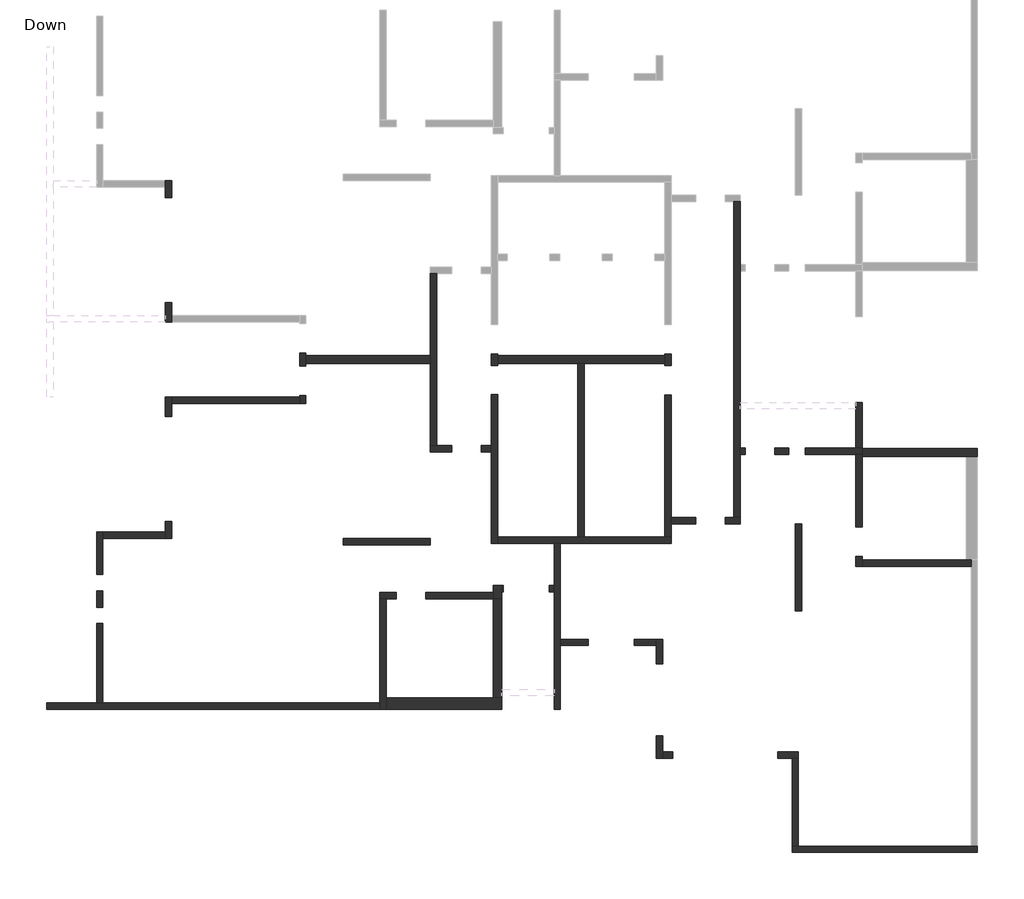
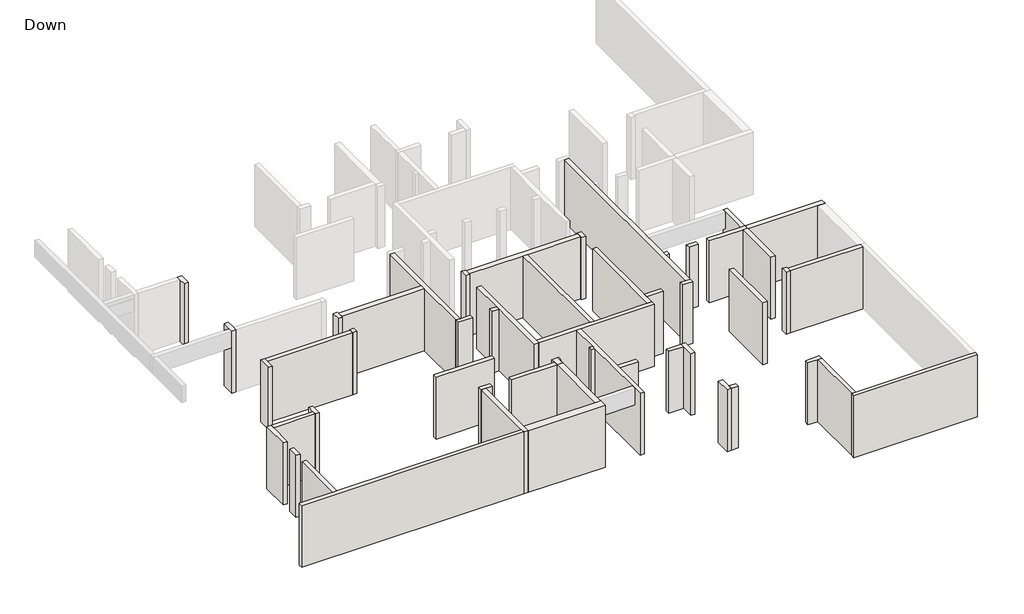
# One storey, part 1 of 2: 53 walls.
"""IFC4 building model written with IfcOpenShell, lengths in millimetres."""

from ifc_helpers import new_model, si_unit, origin, place, context, project, spatial, faceted_brep, element, save

model = new_model("IFC4")

# Units and contexts
model_context = context("Model", 3, world=origin())
ifc_project = project(units=[si_unit("LENGTHUNIT", "METRE", prefix="MILLI")], contexts=[model_context])

# Site, building, storey
site = spatial("IfcSite", under=ifc_project)
building = spatial("IfcBuilding", under=site)
storey = spatial("IfcBuildingStorey", under=building, Name="Down", Elevation=0.0)

# Walls
placement = place(None, origin())
element("IfcWall", 1, ObjectType="19", at=placement, inside=storey, context=model_context, shape_type="Brep", body=[
    faceted_brep([(7776.7577342, 20248.0459905, 0.0), (7776.7577342, 20058.0459905, 0.0), (7776.7577342, 19727.6893828, 0.0), (7776.7577342, 19727.6893828, 2810.0), (7776.7577342, 19727.6893828, 3000.0), (7776.7577342, 20058.0459905, 3000.0), (7776.7577342, 20248.0459905, 3000.0), (7966.7577342, 20248.0459905, 0.0), (7966.7577342, 20248.0459905, 2810.0), (7966.7577342, 20248.0459905, 3000.0), (7966.7577342, 19727.6893828, 3000.0), (7966.7577342, 19727.6893828, 2810.0), (7966.7577342, 19727.6893828, 0.0)], [[[0, 1, 2, 3, 4, 5, 6]], [[7, 8, 9, 10, 11, 12]], [[2, 1, 0, 7, 12]], [[4, 3, 2, 12, 11, 10]], [[6, 5, 4, 10, 9]], [[0, 6, 9, 8, 7]]]),
])
element("IfcWall", 2, ObjectType="19", at=placement, inside=storey, context=model_context, shape_type="Brep", body=[
    faceted_brep([(7776.7577342, 16527.889163, 0.0), (7776.7577342, 15926.4707233, 0.0), (7776.7577342, 15926.4707233, 3000.0), (7776.7577342, 16126.4707233, 3000.0), (7776.7577342, 16527.889163, 3000.0), (7776.7577342, 16527.889163, 2810.0), (7966.7577342, 16527.889163, 0.0), (7966.7577342, 16527.889163, 2810.0), (7966.7577342, 16527.889163, 3000.0), (7966.7577342, 16126.4707233, 3000.0), (7966.7577342, 15926.4707233, 3000.0), (7966.7577342, 15926.4707233, 0.0), (7966.7577342, 16126.4707233, 0.0)], [[[0, 1, 2, 3, 4, 5]], [[6, 7, 8, 9, 10, 11, 12]], [[1, 0, 6, 12, 11]], [[4, 3, 2, 10, 9, 8]], [[0, 5, 4, 8, 7, 6]], [[2, 1, 11, 10]]]),
])
element("IfcWall", 3, ObjectType="19", at=placement, inside=storey, context=model_context, shape_type="Brep", body=[
    faceted_brep([(11878.6856136, 14975.6366408, 0.0), (11878.6856136, 14585.9852573, 0.0), (11878.6856136, 14585.9852573, 2810.0), (11878.6856136, 14585.9852573, 3000.0), (11878.6856136, 14975.6366408, 3000.0), (11878.6856136, 14975.6366408, 2810.0), (12068.6856136, 14975.6366408, 0.0), (12068.6856136, 14975.6366408, 2810.0), (12068.6856136, 14975.6366408, 3000.0), (12068.6856136, 14905.7535122, 3000.0), (12068.6856136, 14655.7535122, 3000.0), (12068.6856136, 14585.9852573, 3000.0), (12068.6856136, 14585.9852573, 2810.0), (12068.6856136, 14585.9852573, 0.0), (12068.6856136, 14655.7535122, 0.0), (12068.6856136, 14905.7535122, 0.0)], [[[0, 1, 2, 3, 4, 5]], [[6, 7, 8, 9, 10, 11, 12, 13, 14, 15]], [[1, 0, 6, 15, 14, 13]], [[3, 2, 1, 13, 12, 11]], [[4, 3, 11, 10, 9, 8]], [[0, 5, 4, 8, 7, 6]]]),
])
element("IfcWall", 4, ObjectType="19", at=placement, inside=storey, context=model_context, shape_type="Brep", body=[
    faceted_brep([(32597.3840453, -100.765317, 0.0), (32407.3840453, -100.765317, 0.0), (27124.7329615, -100.765317, 0.0), (26934.7329615, -100.765317, 0.0), (26934.7329615, -100.765317, 3000.0), (27124.7329615, -100.765317, 3000.0), (32407.3840453, -100.765317, 3000.0), (32597.3840453, -100.765317, 3000.0), (32597.3840453, -290.765317, 0.0), (32597.3840453, -290.765317, 3000.0), (26934.7329615, -290.765317, 3000.0), (26934.7329615, -290.765317, 2810.0), (26934.7329615, -290.765317, 0.0)], [[[0, 1, 2, 3, 4, 5, 6, 7]], [[8, 9, 10, 11, 12]], [[3, 2, 1, 0, 8, 12]], [[7, 6, 5, 4, 10, 9]], [[4, 3, 12, 11, 10]], [[0, 7, 9, 8]]]),
])
element("IfcWall", 5, ObjectType="19", at=placement, inside=storey, context=model_context, shape_type="Brep", body=[
    faceted_brep([(14329.4188071, 4280.8870961, 0.0), (5866.0285364, 4280.8870961, 0.0), (5676.0285364, 4280.8870961, 0.0), (4143.9417549, 4280.8870961, 0.0), (4143.9417549, 4280.8870961, 3000.0), (4344.3623691, 4280.8870961, 3000.0), (5676.0285364, 4280.8870961, 3000.0), (5866.0285364, 4280.8870961, 3000.0), (14329.4188071, 4280.8870961, 3000.0), (14329.4188071, 4280.8870961, 2810.0), (14329.4188071, 4090.8870961, 0.0), (14329.4188071, 4090.8870961, 3000.0), (4143.9417549, 4090.8870961, 3000.0), (4143.9417549, 4090.8870961, 0.0)], [[[0, 1, 2, 3, 4, 5, 6, 7, 8, 9]], [[10, 11, 12, 13]], [[3, 2, 1, 0, 10, 13]], [[4, 3, 13, 12]], [[8, 7, 6, 5, 4, 12, 11]], [[0, 9, 8, 11, 10]]]),
])
element("IfcWall", 6, ObjectType="19", at=placement, inside=storey, context=model_context, shape_type="Brep", body=[
    faceted_brep([(5866.0285364, 4280.8870961, 0.0), (5866.0285364, 6709.6372401, 0.0), (5866.0285364, 6709.6372401, 2810.0), (5866.0285364, 6709.6372401, 3000.0), (5866.0285364, 4280.8870961, 3000.0), (5866.0285364, 4280.8870961, 2810.0), (5676.0285364, 4280.8870961, 0.0), (5676.0285364, 4280.8870961, 2810.0), (5676.0285364, 4280.8870961, 3000.0), (5676.0285364, 6709.6372401, 3000.0), (5676.0285364, 6709.6372401, 2810.0), (5676.0285364, 6709.6372401, 0.0)], [[[0, 1, 2, 3, 4, 5]], [[6, 7, 8, 9, 10, 11]], [[1, 0, 6, 11]], [[3, 2, 1, 11, 10, 9]], [[4, 3, 9, 8]], [[0, 5, 4, 8, 7, 6]]]),
])
element("IfcWall", 7, ObjectType="19", at=placement, inside=storey, context=model_context, shape_type="Brep", body=[
    faceted_brep([(5866.0285364, 7208.8680094, 0.0), (5866.0285364, 7708.0987786, 0.0), (5866.0285364, 7708.0987786, 2810.0), (5866.0285364, 7708.0987786, 3000.0), (5866.0285364, 7208.8680094, 3000.0), (5866.0285364, 7208.8680094, 2810.0), (5676.0285364, 7208.8680094, 0.0), (5676.0285364, 7208.8680094, 2810.0), (5676.0285364, 7208.8680094, 3000.0), (5676.0285364, 7708.0987786, 3000.0), (5676.0285364, 7708.0987786, 2810.0), (5676.0285364, 7708.0987786, 0.0)], [[[0, 1, 2, 3, 4, 5]], [[6, 7, 8, 9, 10, 11]], [[1, 0, 6, 11]], [[3, 2, 1, 11, 10, 9]], [[4, 3, 9, 8]], [[0, 5, 4, 8, 7, 6]]]),
])
element("IfcWall", 8, ObjectType="19", at=placement, inside=storey, context=model_context, shape_type="Brep", body=[
    faceted_brep([(5866.0285364, 8207.3295478, 0.0), (5866.0285364, 9313.461034, 0.0), (5866.0285364, 9503.461034, 0.0), (5866.0285364, 9503.461034, 3000.0), (5866.0285364, 9313.461034, 3000.0), (5866.0285364, 8207.3295478, 3000.0), (5866.0285364, 8207.3295478, 2810.0), (5676.0285364, 8207.3295478, 0.0), (5676.0285364, 8207.3295478, 2810.0), (5676.0285364, 8207.3295478, 3000.0), (5676.0285364, 9308.461034, 3000.0), (5676.0285364, 9503.461034, 3000.0), (5676.0285364, 9503.461034, 0.0)], [[[0, 1, 2, 3, 4, 5, 6]], [[7, 8, 9, 10, 11, 12]], [[2, 1, 0, 7, 12]], [[5, 4, 3, 11, 10, 9]], [[0, 6, 5, 9, 8, 7]], [[3, 2, 12, 11]]]),
])
element("IfcWall", 9, ObjectType="19", at=placement, inside=storey, context=model_context, shape_type="Brep", body=[
    faceted_brep([(27124.7329615, -100.765317, 0.0), (27124.7329615, 2589.8569984, 0.0), (27124.7329615, 2589.8569984, 3000.0), (27124.7329615, -100.765317, 3000.0), (27124.7329615, -100.765317, 2810.0), (26934.7329615, -100.765317, 0.0), (26934.7329615, -100.765317, 3000.0), (26934.7329615, 2589.8569984, 3000.0), (26934.7329615, 2589.8569984, 2810.0), (26934.7329615, 2589.8569984, 0.0)], [[[0, 1, 2, 3, 4]], [[5, 6, 7, 8, 9]], [[1, 0, 5, 9]], [[3, 2, 7, 6]], [[0, 4, 3, 6, 5]], [[2, 1, 9, 8, 7]]]),
])
element("IfcWall", 10, ObjectType="19", at=placement, inside=storey, context=model_context, shape_type="Brep", body=[
    faceted_brep([(27124.7329615, 2779.8569984, 0.0), (26490.0221434, 2779.8569984, 0.0), (26490.0221434, 2779.8569984, 2810.0), (26490.0221434, 2779.8569984, 3000.0), (27124.7329615, 2779.8569984, 3000.0), (27124.7329615, 2779.8569984, 2810.0), (27124.7329615, 2589.8569984, 0.0), (27124.7329615, 2589.8569984, 3000.0), (26934.7329615, 2589.8569984, 3000.0), (26490.0221434, 2589.8569984, 3000.0), (26490.0221434, 2589.8569984, 2810.0), (26490.0221434, 2589.8569984, 0.0), (26934.7329615, 2589.8569984, 0.0)], [[[0, 1, 2, 3, 4, 5]], [[6, 7, 8, 9, 10, 11, 12]], [[1, 0, 6, 12, 11]], [[3, 2, 1, 11, 10, 9]], [[4, 3, 9, 8, 7]], [[0, 5, 4, 7, 6]]]),
])
element("IfcWall", 11, ObjectType="19", at=placement, inside=storey, context=model_context, shape_type="Brep", body=[
    faceted_brep([(23288.1042531, 2779.8569984, 0.0), (22974.0986592, 2779.8569984, 0.0), (22974.0986592, 2779.8569984, 2810.0), (22974.0986592, 2779.8569984, 3000.0), (23288.1042531, 2779.8569984, 3000.0), (23288.1042531, 2779.8569984, 2810.0), (23288.1042531, 2589.8569984, 0.0), (23288.1042531, 2589.8569984, 2810.0), (23288.1042531, 2589.8569984, 3000.0), (22974.0986592, 2589.8569984, 3000.0), (22974.0986592, 2589.8569984, 0.0)], [[[0, 1, 2, 3, 4, 5]], [[6, 7, 8, 9, 10]], [[1, 0, 6, 10]], [[4, 3, 9, 8]], [[0, 5, 4, 8, 7, 6]], [[3, 2, 1, 10, 9]]]),
])
element("IfcWall", 12, ObjectType="19", at=placement, inside=storey, context=model_context, shape_type="Brep", body=[
    faceted_brep([(22974.0986592, 2589.8569984, 0.0), (22974.0986592, 2779.8569984, 0.0), (22974.0986592, 3279.6272511, 0.0), (22974.0986592, 3279.6272511, 2810.0), (22974.0986592, 3279.6272511, 3000.0), (22974.0986592, 2779.8569984, 3000.0), (22974.0986592, 2589.8569984, 3000.0), (22784.0986592, 2589.8569984, 0.0), (22784.0986592, 2589.8569984, 2810.0), (22784.0986592, 2589.8569984, 3000.0), (22784.0986592, 3279.6272511, 3000.0), (22784.0986592, 3279.6272511, 2810.0), (22784.0986592, 3279.6272511, 0.0)], [[[0, 1, 2, 3, 4, 5, 6]], [[7, 8, 9, 10, 11, 12]], [[2, 1, 0, 7, 12]], [[4, 3, 2, 12, 11, 10]], [[6, 5, 4, 10, 9]], [[0, 6, 9, 8, 7]]]),
])
element("IfcWall", 13, ObjectType="19", at=placement, inside=storey, context=model_context, shape_type="Brep", body=[
    faceted_brep([(22974.6890098, 5479.8869654, 0.0), (22974.6890098, 6231.6600151, 0.0), (22974.6890098, 6231.6600151, 2810.0), (22974.6890098, 6231.6600151, 3000.0), (22974.6890098, 5479.8869654, 3000.0), (22974.6890098, 5479.8869654, 2810.0), (22784.6890098, 5479.8869654, 0.0), (22784.6890098, 5479.8869654, 2810.0), (22784.6890098, 5479.8869654, 3000.0), (22784.6890098, 6041.6600151, 3000.0), (22784.6890098, 6231.6600151, 3000.0), (22784.6890098, 6231.6600151, 0.0), (22784.6890098, 6041.6600151, 0.0)], [[[0, 1, 2, 3, 4, 5]], [[6, 7, 8, 9, 10, 11, 12]], [[1, 0, 6, 12, 11]], [[4, 3, 10, 9, 8]], [[0, 5, 4, 8, 7, 6]], [[3, 2, 1, 11, 10]]]),
])
element("IfcWall", 14, ObjectType="19", at=placement, inside=storey, context=model_context, shape_type="Brep", body=[
    faceted_brep([(22784.6890098, 6231.6600151, 0.0), (22104.3264087, 6231.6600151, 0.0), (22104.3264087, 6231.6600151, 2810.0), (22104.3264087, 6231.6600151, 3000.0), (22784.6890098, 6231.6600151, 3000.0), (22784.6890098, 6041.6600151, 0.0), (22784.6890098, 6041.6600151, 2810.0), (22784.6890098, 6041.6600151, 3000.0), (22104.3264087, 6041.6600151, 3000.0), (22104.3264087, 6041.6600151, 2810.0), (22104.3264087, 6041.6600151, 0.0)], [[[0, 1, 2, 3, 4]], [[5, 6, 7, 8, 9, 10]], [[1, 0, 5, 10]], [[3, 2, 1, 10, 9, 8]], [[4, 3, 8, 7]], [[0, 4, 7, 6, 5]]]),
])
element("IfcWall", 15, ObjectType="19", at=placement, inside=storey, context=model_context, shape_type="Brep", body=[
    faceted_brep([(20702.4284964, 6231.6600151, 0.0), (19852.6522503, 6231.6600151, 0.0), (19852.6522503, 6231.6600151, 2810.0), (19852.6522503, 6231.6600151, 3000.0), (20702.4284964, 6231.6600151, 3000.0), (20702.4284964, 6231.6600151, 2810.0), (20702.4284964, 6041.6600151, 0.0), (20702.4284964, 6041.6600151, 2810.0), (20702.4284964, 6041.6600151, 3000.0), (19852.6522503, 6041.6600151, 3000.0), (19852.6522503, 6041.6600151, 2810.0), (19852.6522503, 6041.6600151, 0.0)], [[[0, 1, 2, 3, 4, 5]], [[6, 7, 8, 9, 10, 11]], [[1, 0, 6, 11]], [[4, 3, 9, 8]], [[0, 5, 4, 8, 7, 6]], [[3, 2, 1, 11, 10, 9]]]),
])
element("IfcWall", 16, ObjectType="19", at=placement, inside=storey, context=model_context, shape_type="Brep", body=[
    faceted_brep([(19662.6522503, 9151.9277206, 0.0), (19662.6522503, 7872.8547009, 0.0), (19662.6522503, 7682.8547009, 0.0), (19662.6522503, 4090.6950765, 0.0), (19662.6522503, 4090.6950765, 2810.0), (19662.6522503, 4090.6950765, 3000.0), (19662.6522503, 4692.2283899, 3000.0), (19662.6522503, 7682.8547009, 3000.0), (19662.6522503, 7872.8547009, 3000.0), (19662.6522503, 9151.9277206, 3000.0), (19662.6522503, 9151.9277206, 2810.0), (19852.6522503, 9151.9277206, 0.0), (19852.6522503, 9151.9277206, 2810.0), (19852.6522503, 9151.9277206, 3000.0), (19852.6522503, 6231.6600151, 3000.0), (19852.6522503, 6041.6600151, 3000.0), (19852.6522503, 4090.6950765, 3000.0), (19852.6522503, 4090.6950765, 2810.0), (19852.6522503, 4090.6950765, 0.0), (19852.6522503, 6041.6600151, 0.0), (19852.6522503, 6231.6600151, 0.0)], [[[0, 1, 2, 3, 4, 5, 6, 7, 8, 9, 10]], [[11, 12, 13, 14, 15, 16, 17, 18, 19, 20]], [[3, 2, 1, 0, 11, 20, 19, 18]], [[5, 4, 3, 18, 17, 16]], [[9, 8, 7, 6, 5, 16, 15, 14, 13]], [[0, 10, 9, 13, 12, 11]]]),
])
element("IfcWall", 17, ObjectType="19", at=placement, inside=storey, context=model_context, shape_type="Brep", body=[
    faceted_brep([(5866.0285364, 9313.461034, 0.0), (7776.7577342, 9313.461034, 0.0), (7776.7577342, 9313.461034, 3000.0), (5866.0285364, 9313.461034, 3000.0), (5866.0285364, 9313.461034, 2810.0), (5866.0285364, 9503.461034, 0.0), (5866.0285364, 9503.461034, 3000.0), (7776.7577342, 9503.461034, 3000.0), (7776.7577342, 9503.461034, 2810.0), (7776.7577342, 9503.461034, 0.0)], [[[0, 1, 2, 3, 4]], [[5, 6, 7, 8, 9]], [[1, 0, 5, 9]], [[3, 2, 7, 6]], [[0, 4, 3, 6, 5]], [[2, 1, 9, 8, 7]]]),
])
element("IfcWall", 18, ObjectType="19", at=placement, inside=storey, context=model_context, shape_type="Brep", body=[
    faceted_brep([(7966.7577342, 9313.461034, 0.0), (7966.7577342, 9833.8176417, 0.0), (7966.7577342, 9833.8176417, 2810.0), (7966.7577342, 9833.8176417, 3000.0), (7966.7577342, 9313.461034, 3000.0), (7966.7577342, 9313.461034, 2810.0), (7776.7577342, 9313.461034, 0.0), (7776.7577342, 9313.461034, 3000.0), (7776.7577342, 9503.461034, 3000.0), (7776.7577342, 9833.8176417, 3000.0), (7776.7577342, 9833.8176417, 2810.0), (7776.7577342, 9833.8176417, 0.0), (7776.7577342, 9503.461034, 0.0)], [[[0, 1, 2, 3, 4, 5]], [[6, 7, 8, 9, 10, 11, 12]], [[1, 0, 6, 12, 11]], [[3, 2, 1, 11, 10, 9]], [[4, 3, 9, 8, 7]], [[0, 5, 4, 7, 6]]]),
])
element("IfcWall", 19, ObjectType="19", at=placement, inside=storey, context=model_context, shape_type="Brep", body=[
    faceted_brep([(7966.7577342, 13033.6178615, 0.0), (7966.7577342, 13435.0363012, 0.0), (7966.7577342, 13635.0363012, 0.0), (7966.7577342, 13635.0363012, 3000.0), (7966.7577342, 13435.0363012, 3000.0), (7966.7577342, 13033.6178615, 3000.0), (7966.7577342, 13033.6178615, 2810.0), (7776.7577342, 13033.6178615, 0.0), (7776.7577342, 13033.6178615, 2810.0), (7776.7577342, 13033.6178615, 3000.0), (7776.7577342, 13435.0363012, 3000.0), (7776.7577342, 13635.0363012, 3000.0), (7776.7577342, 13635.0363012, 0.0)], [[[0, 1, 2, 3, 4, 5, 6]], [[7, 8, 9, 10, 11, 12]], [[2, 1, 0, 7, 12]], [[5, 4, 3, 11, 10, 9]], [[0, 6, 5, 9, 8, 7]], [[3, 2, 12, 11]]]),
])
element("IfcWall", 20, ObjectType="19", at=placement, inside=storey, context=model_context, shape_type="Brep", body=[
    faceted_brep([(12068.6856136, 13435.0363012, 0.0), (12068.6856136, 13683.7427241, 0.0), (12068.6856136, 13683.7427241, 2810.0), (12068.6856136, 13683.7427241, 3000.0), (12068.6856136, 13435.0363012, 3000.0), (12068.6856136, 13435.0363012, 2810.0), (11878.6856136, 13435.0363012, 0.0), (11878.6856136, 13435.0363012, 3000.0), (11878.6856136, 13635.0363012, 3000.0), (11878.6856136, 13683.7427241, 3000.0), (11878.6856136, 13683.7427241, 2810.0), (11878.6856136, 13683.7427241, 0.0), (11878.6856136, 13635.0363012, 0.0)], [[[0, 1, 2, 3, 4, 5]], [[6, 7, 8, 9, 10, 11, 12]], [[1, 0, 6, 12, 11]], [[3, 2, 1, 11, 10, 9]], [[4, 3, 9, 8, 7]], [[0, 5, 4, 7, 6]]]),
])
element("IfcWall", 21, ObjectType="19", at=placement, inside=storey, context=model_context, shape_type="Brep", body=[
    faceted_brep([(18051.1049523, 7682.8547009, 0.0), (18101.9290458, 7682.8547009, 0.0), (18101.9290458, 7682.8547009, 2810.0), (18101.9290458, 7682.8547009, 3000.0), (18051.1049523, 7682.8547009, 3000.0), (18051.1049523, 7682.8547009, 2810.0), (18051.1049523, 7872.8547009, 0.0), (18051.1049523, 7872.8547009, 3000.0), (18101.9290458, 7872.8547009, 3000.0), (18101.9290458, 7872.8547009, 2810.0), (18101.9290458, 7872.8547009, 0.0)], [[[0, 1, 2, 3, 4, 5]], [[6, 7, 8, 9, 10]], [[1, 0, 6, 10]], [[3, 2, 1, 10, 9, 8]], [[4, 3, 8, 7]], [[0, 5, 4, 7, 6]]]),
])
element("IfcWall", 22, ObjectType="19", at=placement, inside=storey, context=model_context, shape_type="Brep", body=[
    faceted_brep([(19501.7092875, 7682.8547009, 0.0), (19662.6522503, 7682.8547009, 0.0), (19662.6522503, 7682.8547009, 2810.0), (19662.6522503, 7682.8547009, 3000.0), (19501.7092875, 7682.8547009, 3000.0), (19501.7092875, 7682.8547009, 2810.0), (19501.7092875, 7872.8547009, 0.0), (19501.7092875, 7872.8547009, 2810.0), (19501.7092875, 7872.8547009, 3000.0), (19662.6522503, 7872.8547009, 3000.0), (19662.6522503, 7872.8547009, 2810.0), (19662.6522503, 7872.8547009, 0.0)], [[[0, 1, 2, 3, 4, 5]], [[6, 7, 8, 9, 10, 11]], [[1, 0, 6, 11]], [[4, 3, 9, 8]], [[0, 5, 4, 8, 7, 6]], [[3, 2, 1, 11, 10, 9]]]),
])
element("IfcWall", 23, ObjectType="20", at=placement, inside=storey, context=model_context, shape_type="Brep", body=[
    faceted_brep([(23033.0448184, 14956.5776057, 0.0), (23033.0448184, 14905.8683859, 0.0), (23033.0448184, 14655.8683859, 0.0), (23033.0448184, 14596.5776057, 0.0), (23033.0448184, 14596.5776057, 2810.0), (23033.0448184, 14596.5776057, 3000.0), (23033.0448184, 14655.8683859, 3000.0), (23033.0448184, 14905.8683859, 3000.0), (23033.0448184, 14956.5776057, 3000.0), (23033.0448184, 14956.5776057, 2810.0), (23233.0448184, 14956.5776057, 0.0), (23233.0448184, 14956.5776057, 2810.0), (23233.0448184, 14956.5776057, 3000.0), (23233.0448184, 14596.5776057, 3000.0), (23233.0448184, 14596.5776057, 2810.0), (23233.0448184, 14596.5776057, 0.0)], [[[0, 1, 2, 3, 4, 5, 6, 7, 8, 9]], [[10, 11, 12, 13, 14, 15]], [[3, 2, 1, 0, 10, 15]], [[5, 4, 3, 15, 14, 13]], [[8, 7, 6, 5, 13, 12]], [[0, 9, 8, 12, 11, 10]]]),
])
element("IfcWall", 24, ObjectType="20", at=placement, inside=storey, context=model_context, shape_type="Brep", body=[
    faceted_brep([(17931.3366974, 14607.1619629, 0.0), (17931.3366974, 14655.8683859, 0.0), (17931.3366974, 14905.8683859, 0.0), (17931.3366974, 14956.5776057, 0.0), (17931.3366974, 14956.5776057, 2810.0), (17931.3366974, 14956.5776057, 3000.0), (17931.3366974, 14905.8683859, 3000.0), (17931.3366974, 14655.8683859, 3000.0), (17931.3366974, 14607.1619629, 3000.0), (17931.3366974, 14607.1619629, 2810.0), (17731.3366974, 14607.1619629, 0.0), (17731.3366974, 14607.1619629, 2810.0), (17731.3366974, 14607.1619629, 3000.0), (17731.3366974, 14956.5776057, 3000.0), (17731.3366974, 14956.5776057, 2810.0), (17731.3366974, 14956.5776057, 0.0)], [[[0, 1, 2, 3, 4, 5, 6, 7, 8, 9]], [[10, 11, 12, 13, 14, 15]], [[3, 2, 1, 0, 10, 15]], [[5, 4, 3, 15, 14, 13]], [[8, 7, 6, 5, 13, 12]], [[0, 9, 8, 12, 11, 10]]]),
])
element("IfcWall", 25, ObjectType="20", at=placement, inside=storey, context=model_context, shape_type="Brep", body=[
    faceted_brep([(14329.4188071, 7461.0876447, 0.0), (14329.4188071, 4280.8870961, 0.0), (14329.4188071, 4090.8870961, 0.0), (14329.4188071, 4090.8870961, 3000.0), (14329.4188071, 4280.8870961, 3000.0), (14329.4188071, 7461.0876447, 3000.0), (14529.4188071, 7461.0876447, 0.0), (14529.4188071, 7461.0876447, 2810.0), (14529.4188071, 7461.0876447, 3000.0), (14529.4188071, 4440.7910863, 3000.0), (14529.4188071, 4090.8870961, 3000.0), (14529.4188071, 4090.8870961, 0.0), (14529.4188071, 4440.7910863, 0.0)], [[[0, 1, 2, 3, 4, 5]], [[6, 7, 8, 9, 10, 11, 12]], [[2, 1, 0, 6, 12, 11]], [[5, 4, 3, 10, 9, 8]], [[3, 2, 11, 10]], [[0, 5, 8, 7, 6]]]),
])
element("IfcWall", 26, ObjectType="20", at=placement, inside=storey, context=model_context, shape_type="Brep", body=[
    faceted_brep([(29076.6368672, 8461.5671173, 0.0), (32407.3840453, 8461.5671173, 0.0), (32407.3840453, 8461.5671173, 2810.0), (32407.3840453, 8461.5671173, 3000.0), (29076.6368672, 8461.5671173, 3000.0), (29076.6368672, 8661.5671173, 0.0), (29076.6368672, 8661.5671173, 2810.0), (29076.6368672, 8661.5671173, 3000.0), (32247.3840453, 8661.5671173, 3000.0), (32407.3840453, 8661.5671173, 3000.0), (32407.3840453, 8661.5671173, 0.0), (32247.3840453, 8661.5671173, 0.0)], [[[0, 1, 2, 3, 4]], [[5, 6, 7, 8, 9, 10, 11]], [[1, 0, 5, 11, 10]], [[4, 3, 9, 8, 7]], [[3, 2, 1, 10, 9]], [[0, 4, 7, 6, 5]]]),
])
element("IfcWall", 27, ObjectType="20", at=placement, inside=storey, context=model_context, shape_type="Brep", body=[
    faceted_brep([(7966.7577342, 13435.0363012, 0.0), (11878.6856136, 13435.0363012, 0.0), (11878.6856136, 13435.0363012, 3000.0), (7966.7577342, 13435.0363012, 3000.0), (7966.7577342, 13435.0363012, 2810.0), (7966.7577342, 13635.0363012, 0.0), (7966.7577342, 13635.0363012, 3000.0), (11878.6856136, 13635.0363012, 3000.0), (11878.6856136, 13635.0363012, 0.0)], [[[0, 1, 2, 3, 4]], [[5, 6, 7, 8]], [[1, 0, 5, 8]], [[3, 2, 7, 6]], [[0, 4, 3, 6, 5]], [[2, 1, 8, 7]]]),
])
element("IfcWall", 28, ObjectType="20", at=placement, inside=storey, context=model_context, shape_type="Brep", body=[
    faceted_brep([(14329.4188071, 7461.0876447, 0.0), (14529.4188071, 7461.0876447, 0.0), (14830.1280269, 7461.0876447, 0.0), (14830.1280269, 7461.0876447, 2810.0), (14830.1280269, 7461.0876447, 3000.0), (14529.4188071, 7461.0876447, 3000.0), (14329.4188071, 7461.0876447, 3000.0), (14329.4188071, 7661.0876447, 0.0), (14329.4188071, 7661.0876447, 2810.0), (14329.4188071, 7661.0876447, 3000.0), (14830.1280269, 7661.0876447, 3000.0), (14830.1280269, 7661.0876447, 2810.0), (14830.1280269, 7661.0876447, 0.0)], [[[0, 1, 2, 3, 4, 5, 6]], [[7, 8, 9, 10, 11, 12]], [[2, 1, 0, 7, 12]], [[4, 3, 2, 12, 11, 10]], [[6, 5, 4, 10, 9]], [[0, 6, 9, 8, 7]]]),
])
element("IfcWall", 29, ObjectType="20", at=placement, inside=storey, context=model_context, shape_type="Brep", body=[
    faceted_brep([(15730.1380159, 7461.0876447, 0.0), (17801.1049523, 7461.0876447, 0.0), (17801.1049523, 7461.0876447, 2810.0), (17801.1049523, 7461.0876447, 3000.0), (15730.1380159, 7461.0876447, 3000.0), (15730.1380159, 7461.0876447, 2810.0), (15730.1380159, 7661.0876447, 0.0), (15730.1380159, 7661.0876447, 2810.0), (15730.1380159, 7661.0876447, 3000.0), (17801.1049523, 7661.0876447, 3000.0), (17801.1049523, 7661.0876447, 2810.0), (17801.1049523, 7661.0876447, 0.0)], [[[0, 1, 2, 3, 4, 5]], [[6, 7, 8, 9, 10, 11]], [[1, 0, 6, 11]], [[4, 3, 9, 8]], [[0, 5, 4, 8, 7, 6]], [[3, 2, 1, 11, 10, 9]]]),
])
element("IfcWall", 30, ObjectType="20", at=placement, inside=storey, context=model_context, shape_type="Brep", body=[
    faceted_brep([(13218.5807289, 9112.8706834, 0.0), (15869.904273, 9112.8706834, 0.0), (15869.904273, 9112.8706834, 2810.0), (15869.904273, 9112.8706834, 3000.0), (13218.5807289, 9112.8706834, 3000.0), (13218.5807289, 9112.8706834, 2810.0), (13218.5807289, 9312.8706834, 0.0), (13218.5807289, 9312.8706834, 2810.0), (13218.5807289, 9312.8706834, 3000.0), (15869.904273, 9312.8706834, 3000.0), (15869.904273, 9312.8706834, 2810.0), (15869.904273, 9312.8706834, 0.0)], [[[0, 1, 2, 3, 4, 5]], [[6, 7, 8, 9, 10, 11]], [[1, 0, 6, 11]], [[3, 2, 1, 11, 10, 9]], [[4, 3, 9, 8]], [[0, 5, 4, 8, 7, 6]]]),
])
element("IfcWall", 31, ObjectType="20", at=placement, inside=storey, context=model_context, shape_type="Brep", body=[
    faceted_brep([(15871.0829765, 17407.9011498, 0.0), (15871.0829765, 14905.7535122, 0.0), (15871.0829765, 14655.7535122, 0.0), (15871.0829765, 12153.6058746, 0.0), (15871.0829765, 12153.6058746, 3000.0), (15871.0829765, 14655.7535122, 3000.0), (15871.0829765, 14905.7535122, 3000.0), (15871.0829765, 17407.9011498, 3000.0), (16071.0829765, 17407.9011498, 0.0), (16071.0829765, 17407.9011498, 2810.0), (16071.0829765, 17407.9011498, 3000.0), (16071.0829765, 12153.6058746, 3000.0), (16071.0829765, 12153.6058746, 2810.0), (16071.0829765, 12153.6058746, 0.0)], [[[0, 1, 2, 3, 4, 5, 6, 7]], [[8, 9, 10, 11, 12, 13]], [[3, 2, 1, 0, 8, 13]], [[7, 6, 5, 4, 11, 10]], [[4, 3, 13, 12, 11]], [[0, 7, 10, 9, 8]]]),
])
element("IfcWall", 32, ObjectType="20", at=placement, inside=storey, context=model_context, shape_type="Brep", body=[
    faceted_brep([(15871.0829765, 11953.6058746, 0.0), (16530.6174885, 11953.6058746, 0.0), (16530.6174885, 11953.6058746, 2810.0), (16530.6174885, 11953.6058746, 3000.0), (15871.0829765, 11953.6058746, 3000.0), (15871.0829765, 11953.6058746, 2810.0), (15871.0829765, 12153.6058746, 0.0), (15871.0829765, 12153.6058746, 3000.0), (16071.0829765, 12153.6058746, 3000.0), (16530.6174885, 12153.6058746, 3000.0), (16530.6174885, 12153.6058746, 2810.0), (16530.6174885, 12153.6058746, 0.0), (16071.0829765, 12153.6058746, 0.0)], [[[0, 1, 2, 3, 4, 5]], [[6, 7, 8, 9, 10, 11, 12]], [[1, 0, 6, 12, 11]], [[3, 2, 1, 11, 10, 9]], [[4, 3, 9, 8, 7]], [[0, 5, 4, 7, 6]]]),
])
element("IfcWall", 33, ObjectType="20", at=placement, inside=storey, context=model_context, shape_type="Brep", body=[
    faceted_brep([(17430.6274775, 11953.6058746, 0.0), (17731.3366974, 11953.6058746, 0.0), (17731.3366974, 11953.6058746, 2810.0), (17731.3366974, 11953.6058746, 3000.0), (17430.6274775, 11953.6058746, 3000.0), (17430.6274775, 11953.6058746, 2810.0), (17430.6274775, 12153.6058746, 0.0), (17430.6274775, 12153.6058746, 2810.0), (17430.6274775, 12153.6058746, 3000.0), (17731.3366974, 12153.6058746, 3000.0), (17731.3366974, 12153.6058746, 2810.0), (17731.3366974, 12153.6058746, 0.0)], [[[0, 1, 2, 3, 4, 5]], [[6, 7, 8, 9, 10, 11]], [[1, 0, 6, 11]], [[4, 3, 9, 8]], [[0, 5, 4, 8, 7, 6]], [[3, 2, 1, 11, 10, 9]]]),
])
element("IfcWall", 34, ObjectType="20", at=placement, inside=storey, context=model_context, shape_type="Brep", body=[
    faceted_brep([(17731.3366974, 13708.6058746, 0.0), (17731.3366974, 12153.6058746, 0.0), (17731.3366974, 11953.6058746, 0.0), (17731.3366974, 9151.9277206, 0.0), (17731.3366974, 9151.9277206, 2810.0), (17731.3366974, 9151.9277206, 3000.0), (17731.3366974, 11953.6058746, 3000.0), (17731.3366974, 12153.6058746, 3000.0), (17731.3366974, 13708.6058746, 3000.0), (17731.3366974, 13708.6058746, 2810.0), (17931.3366974, 13708.6058746, 0.0), (17931.3366974, 13708.6058746, 3000.0), (17931.3366974, 9351.9277206, 3000.0), (17931.3366974, 9151.9277206, 3000.0), (17931.3366974, 9151.9277206, 0.0), (17931.3366974, 9351.9277206, 0.0)], [[[0, 1, 2, 3, 4, 5, 6, 7, 8, 9]], [[10, 11, 12, 13, 14, 15]], [[3, 2, 1, 0, 10, 15, 14]], [[8, 7, 6, 5, 13, 12, 11]], [[0, 9, 8, 11, 10]], [[5, 4, 3, 14, 13]]]),
])
element("IfcWall", 35, ObjectType="20", at=placement, inside=storey, context=model_context, shape_type="Brep", body=[
    faceted_brep([(17931.3366974, 9151.9277206, 0.0), (19662.6522503, 9151.9277206, 0.0), (19852.6522503, 9151.9277206, 0.0), (23233.0448184, 9151.9277206, 0.0), (23233.0448184, 9151.9277206, 2810.0), (23233.0448184, 9151.9277206, 3000.0), (19852.6522503, 9151.9277206, 3000.0), (19662.6522503, 9151.9277206, 3000.0), (17931.3366974, 9151.9277206, 3000.0), (17931.3366974, 9351.9277206, 0.0), (17931.3366974, 9351.9277206, 3000.0), (20384.2581025, 9351.9277206, 3000.0), (20584.2581025, 9351.9277206, 3000.0), (23033.0448184, 9351.9277206, 3000.0), (23233.0448184, 9351.9277206, 3000.0), (23233.0448184, 9351.9277206, 0.0), (23033.0448184, 9351.9277206, 0.0), (20584.2581025, 9351.9277206, 0.0), (20384.2581025, 9351.9277206, 0.0)], [[[0, 1, 2, 3, 4, 5, 6, 7, 8]], [[9, 10, 11, 12, 13, 14, 15, 16, 17, 18]], [[3, 2, 1, 0, 9, 18, 17, 16, 15]], [[8, 7, 6, 5, 14, 13, 12, 11, 10]], [[0, 8, 10, 9]], [[5, 4, 3, 15, 14]]]),
])
element("IfcWall", 36, ObjectType="20", at=placement, inside=storey, context=model_context, shape_type="Brep", body=[
    faceted_brep([(23233.0448184, 9752.4071932, 0.0), (23984.8178681, 9752.4071932, 0.0), (23984.8178681, 9752.4071932, 2810.0), (23984.8178681, 9752.4071932, 3000.0), (23233.0448184, 9752.4071932, 3000.0), (23233.0448184, 9752.4071932, 2810.0), (23233.0448184, 9952.4071932, 0.0), (23233.0448184, 9952.4071932, 2810.0), (23233.0448184, 9952.4071932, 3000.0), (23984.8178681, 9952.4071932, 3000.0), (23984.8178681, 9952.4071932, 2810.0), (23984.8178681, 9952.4071932, 0.0)], [[[0, 1, 2, 3, 4, 5]], [[6, 7, 8, 9, 10, 11]], [[1, 0, 6, 11]], [[3, 2, 1, 11, 10, 9]], [[4, 3, 9, 8]], [[0, 5, 4, 8, 7, 6]]]),
])
element("IfcWall", 37, ObjectType="20", at=placement, inside=storey, context=model_context, shape_type="Brep", body=[
    faceted_brep([(24884.8278571, 9752.4071932, 0.0), (25344.8278571, 9752.4071932, 0.0), (25344.8278571, 9752.4071932, 2810.0), (25344.8278571, 9752.4071932, 3000.0), (24884.8278571, 9752.4071932, 3000.0), (24884.8278571, 9752.4071932, 2810.0), (24884.8278571, 9952.4071932, 0.0), (24884.8278571, 9952.4071932, 2810.0), (24884.8278571, 9952.4071932, 3000.0), (25144.8278571, 9952.4071932, 3000.0), (25344.8278571, 9952.4071932, 3000.0), (25344.8278571, 9952.4071932, 0.0), (25144.8278571, 9952.4071932, 0.0)], [[[0, 1, 2, 3, 4, 5]], [[6, 7, 8, 9, 10, 11, 12]], [[1, 0, 6, 12, 11]], [[4, 3, 10, 9, 8]], [[0, 5, 4, 8, 7, 6]], [[3, 2, 1, 11, 10]]]),
])
element("IfcWall", 38, ObjectType="20", at=placement, inside=storey, context=model_context, shape_type="Brep", body=[
    faceted_brep([(25344.8278571, 9952.4071932, 0.0), (25344.8278571, 11873.1343933, 0.0), (25344.8278571, 12073.1343933, 0.0), (25344.8278571, 17488.3726312, 0.0), (25344.8278571, 17688.3726312, 0.0), (25344.8278571, 19609.0998313, 0.0), (25344.8278571, 19609.0998313, 3000.0), (25344.8278571, 17688.3726312, 3000.0), (25344.8278571, 17488.3726312, 3000.0), (25344.8278571, 16296.9481981, 3000.0), (25344.8278571, 13264.5588264, 3000.0), (25344.8278571, 12073.1343933, 3000.0), (25344.8278571, 11873.1343933, 3000.0), (25344.8278571, 9952.4071932, 3000.0), (25144.8278571, 9952.4071932, 0.0), (25144.8278571, 9952.4071932, 2810.0), (25144.8278571, 9952.4071932, 3000.0), (25144.8278571, 19609.0998313, 3000.0), (25144.8278571, 19609.0998313, 2810.0), (25144.8278571, 19609.0998313, 0.0)], [[[0, 1, 2, 3, 4, 5, 6, 7, 8, 9, 10, 11, 12, 13]], [[14, 15, 16, 17, 18, 19]], [[5, 4, 3, 2, 1, 0, 14, 19]], [[13, 12, 11, 10, 9, 8, 7, 6, 17, 16]], [[0, 13, 16, 15, 14]], [[6, 5, 19, 18, 17]]]),
])
element("IfcWall", 39, ObjectType="20", at=placement, inside=storey, context=model_context, shape_type="Brep", body=[
    faceted_brep([(23033.0448184, 13704.9194297, 0.0), (23033.0448184, 9351.9277206, 0.0), (23033.0448184, 9351.9277206, 3000.0), (23033.0448184, 13704.9194297, 3000.0), (23233.0448184, 13704.9194297, 0.0), (23233.0448184, 13704.9194297, 2810.0), (23233.0448184, 13704.9194297, 3000.0), (23233.0448184, 9952.4071932, 3000.0), (23233.0448184, 9752.4071932, 3000.0), (23233.0448184, 9351.9277206, 3000.0), (23233.0448184, 9351.9277206, 0.0), (23233.0448184, 9752.4071932, 0.0), (23233.0448184, 9952.4071932, 0.0)], [[[0, 1, 2, 3]], [[4, 5, 6, 7, 8, 9, 10, 11, 12]], [[1, 0, 4, 12, 11, 10]], [[3, 2, 9, 8, 7, 6]], [[0, 3, 6, 5, 4]], [[2, 1, 10, 9]]]),
])
element("IfcWall", 40, ObjectType="20", at=placement, inside=storey, context=model_context, shape_type="Brep", body=[
    faceted_brep([(25344.8278571, 11873.1343933, 0.0), (25494.7169791, 11873.1343933, 0.0), (25494.7169791, 11873.1343933, 2810.0), (25494.7169791, 11873.1343933, 3000.0), (25344.8278571, 11873.1343933, 3000.0), (25344.8278571, 11873.1343933, 2810.0), (25344.8278571, 12073.1343933, 0.0), (25344.8278571, 12073.1343933, 2810.0), (25344.8278571, 12073.1343933, 3000.0), (25494.7169791, 12073.1343933, 3000.0), (25494.7169791, 12073.1343933, 2810.0), (25494.7169791, 12073.1343933, 0.0)], [[[0, 1, 2, 3, 4, 5]], [[6, 7, 8, 9, 10, 11]], [[1, 0, 6, 11]], [[3, 2, 1, 11, 10, 9]], [[4, 3, 9, 8]], [[0, 5, 4, 8, 7, 6]]]),
])
element("IfcWall", 41, ObjectType="20", at=placement, inside=storey, context=model_context, shape_type="Brep", body=[
    faceted_brep([(26394.7269681, 11873.1343933, 0.0), (26824.6140922, 11873.1343933, 0.0), (26824.6140922, 11873.1343933, 2810.0), (26824.6140922, 11873.1343933, 3000.0), (26394.7269681, 11873.1343933, 3000.0), (26394.7269681, 11873.1343933, 2810.0), (26394.7269681, 12073.1343933, 0.0), (26394.7269681, 12073.1343933, 2810.0), (26394.7269681, 12073.1343933, 3000.0), (26824.6140922, 12073.1343933, 3000.0), (26824.6140922, 12073.1343933, 2810.0), (26824.6140922, 12073.1343933, 0.0)], [[[0, 1, 2, 3, 4, 5]], [[6, 7, 8, 9, 10, 11]], [[1, 0, 6, 11]], [[3, 2, 1, 11, 10, 9]], [[4, 3, 9, 8]], [[0, 5, 4, 8, 7, 6]]]),
])
element("IfcWall", 42, ObjectType="20", at=placement, inside=storey, context=model_context, shape_type="Brep", body=[
    faceted_brep([(27326.5020155, 11873.1343933, 0.0), (28876.6368672, 11873.1343933, 0.0), (29075.6979001, 11873.1343933, 0.0), (29075.6979001, 11873.1343933, 3000.0), (28876.6368672, 11873.1343933, 3000.0), (27326.5020155, 11873.1343933, 3000.0), (27326.5020155, 11873.1343933, 2810.0), (27326.5020155, 12073.1343933, 0.0), (27326.5020155, 12073.1343933, 2810.0), (27326.5020155, 12073.1343933, 3000.0), (28875.6979001, 12073.1343933, 3000.0), (29075.6979001, 12073.1343933, 3000.0), (29075.6979001, 12073.1343933, 0.0), (28875.6979001, 12073.1343933, 0.0), (29075.6979001, 12063.7247439, 0.0), (29075.6979001, 12063.7247439, 3000.0)], [[[0, 1, 2, 3, 4, 5, 6]], [[7, 8, 9, 10, 11, 12, 13]], [[2, 1, 0, 7, 13, 12, 14]], [[5, 4, 3, 15, 11, 10, 9]], [[0, 6, 5, 9, 8, 7]], [[3, 2, 14, 12, 11, 15]]]),
])
element("IfcWall", 43, ObjectType="20", at=placement, inside=storey, context=model_context, shape_type="Brep", body=[
    faceted_brep([(29075.6979001, 12073.1343933, 0.0), (29075.6979001, 13465.6226562, 0.0), (29075.6979001, 13465.6226562, 3000.0), (29075.6979001, 12073.1343933, 3000.0), (28875.6979001, 12073.1343933, 0.0), (28875.6979001, 12073.1343933, 2810.0), (28875.6979001, 12073.1343933, 3000.0), (28875.6979001, 13264.5588264, 3000.0), (28875.6979001, 13465.6226562, 3000.0), (28875.6979001, 13465.6226562, 0.0)], [[[0, 1, 2, 3]], [[4, 5, 6, 7, 8, 9]], [[1, 0, 4, 9]], [[2, 1, 9, 8]], [[3, 2, 8, 7, 6]], [[0, 3, 6, 5, 4]]]),
])
element("IfcWall", 44, ObjectType="20", at=placement, inside=storey, context=model_context, shape_type="Brep", body=[
    faceted_brep([(29076.6368672, 8461.5671173, 0.0), (29076.6368672, 8661.5671173, 0.0), (29076.6368672, 8762.2763371, 0.0), (29076.6368672, 8762.2763371, 2810.0), (29076.6368672, 8762.2763371, 3000.0), (29076.6368672, 8661.5671173, 3000.0), (29076.6368672, 8461.5671173, 3000.0), (28876.6368672, 8461.5671173, 0.0), (28876.6368672, 8461.5671173, 2810.0), (28876.6368672, 8461.5671173, 3000.0), (28876.6368672, 8762.2763371, 3000.0), (28876.6368672, 8762.2763371, 2810.0), (28876.6368672, 8762.2763371, 0.0)], [[[0, 1, 2, 3, 4, 5, 6]], [[7, 8, 9, 10, 11, 12]], [[2, 1, 0, 7, 12]], [[4, 3, 2, 12, 11, 10]], [[6, 5, 4, 10, 9]], [[0, 6, 9, 8, 7]]]),
])
element("IfcWall", 45, ObjectType="20", at=placement, inside=storey, context=model_context, shape_type="Brep", body=[
    faceted_brep([(29076.6368672, 9662.2863261, 0.0), (29076.6368672, 11813.7247439, 0.0), (29076.6368672, 11813.7247439, 2810.0), (29076.6368672, 11813.7247439, 3000.0), (29076.6368672, 9662.2863261, 3000.0), (29076.6368672, 9662.2863261, 2810.0), (28876.6368672, 9662.2863261, 0.0), (28876.6368672, 9662.2863261, 2810.0), (28876.6368672, 9662.2863261, 3000.0), (28876.6368672, 11873.1343933, 3000.0), (28876.6368672, 11873.1343933, 2810.0), (28876.6368672, 11873.1343933, 0.0), (29075.6979001, 11873.1343933, 0.0), (29075.6979001, 11813.7247439, 0.0), (29075.6979001, 11813.7247439, 3000.0), (29075.6979001, 11873.1343933, 3000.0)], [[[0, 1, 2, 3, 4, 5]], [[6, 7, 8, 9, 10, 11]], [[1, 0, 6, 11, 12, 13]], [[4, 3, 14, 15, 9, 8]], [[0, 5, 4, 8, 7, 6]], [[3, 2, 1, 13, 14]], [[13, 12, 15, 14]], [[12, 11, 10, 9, 15]]]),
])
element("IfcWall", 46, ObjectType="20", at=placement, inside=storey, context=model_context, shape_type="Brep", body=[
    faceted_brep([(27025.7927957, 9753.3461603, 0.0), (27025.7927957, 7102.0226162, 0.0), (27025.7927957, 7102.0226162, 2810.0), (27025.7927957, 7102.0226162, 3000.0), (27025.7927957, 9753.3461603, 3000.0), (27025.7927957, 9753.3461603, 2810.0), (27225.7927957, 9753.3461603, 0.0), (27225.7927957, 9753.3461603, 2810.0), (27225.7927957, 9753.3461603, 3000.0), (27225.7927957, 7102.0226162, 3000.0), (27225.7927957, 7102.0226162, 2810.0), (27225.7927957, 7102.0226162, 0.0)], [[[0, 1, 2, 3, 4, 5]], [[6, 7, 8, 9, 10, 11]], [[1, 0, 6, 11]], [[3, 2, 1, 11, 10, 9]], [[4, 3, 9, 8]], [[0, 5, 4, 8, 7, 6]]]),
])
element("IfcWall", 47, ObjectType="20", at=placement, inside=storey, context=model_context, shape_type="Brep", body=[
    faceted_brep([(20384.2581025, 14655.8683859, 0.0), (20384.2581025, 9351.9277206, 0.0), (20384.2581025, 9351.9277206, 3000.0), (20384.2581025, 13708.6058746, 3000.0), (20384.2581025, 14655.8683859, 3000.0), (20384.2581025, 14655.8683859, 2810.0), (20584.2581025, 14655.8683859, 0.0), (20584.2581025, 14655.8683859, 2810.0), (20584.2581025, 14655.8683859, 3000.0), (20584.2581025, 13704.9194297, 3000.0), (20584.2581025, 9351.9277206, 3000.0), (20584.2581025, 9351.9277206, 0.0)], [[[0, 1, 2, 3, 4, 5]], [[6, 7, 8, 9, 10, 11]], [[1, 0, 6, 11]], [[4, 3, 2, 10, 9, 8]], [[0, 5, 4, 8, 7, 6]], [[2, 1, 11, 10]]]),
])
element("IfcWall", 48, ObjectType="25", at=placement, inside=storey, context=model_context, shape_type="Brep", body=[
    faceted_brep([(12068.6856136, 14655.7535122, 0.0), (15871.0829765, 14655.7535122, 0.0), (15871.0829765, 14655.7535122, 2810.0), (15871.0829765, 14655.7535122, 3000.0), (12068.6856136, 14655.7535122, 3000.0), (12068.6856136, 14655.7535122, 2810.0), (12068.6856136, 14905.7535122, 0.0), (12068.6856136, 14905.7535122, 2810.0), (12068.6856136, 14905.7535122, 3000.0), (15871.0829765, 14905.7535122, 3000.0), (15871.0829765, 14905.7535122, 2810.0), (15871.0829765, 14905.7535122, 0.0)], [[[0, 1, 2, 3, 4, 5]], [[6, 7, 8, 9, 10, 11]], [[1, 0, 6, 11]], [[4, 3, 9, 8]], [[0, 5, 4, 8, 7, 6]], [[3, 2, 1, 11, 10, 9]]]),
])
element("IfcWall", 49, ObjectType="25", at=placement, inside=storey, context=model_context, shape_type="Brep", body=[
    faceted_brep([(23033.0448184, 14905.8683859, 0.0), (17931.3366974, 14905.8683859, 0.0), (17931.3366974, 14905.8683859, 2810.0), (17931.3366974, 14905.8683859, 3000.0), (23033.0448184, 14905.8683859, 3000.0), (23033.0448184, 14905.8683859, 2810.0), (23033.0448184, 14655.8683859, 0.0), (23033.0448184, 14655.8683859, 2810.0), (23033.0448184, 14655.8683859, 3000.0), (20584.2581025, 14655.8683859, 3000.0), (20384.2581025, 14655.8683859, 3000.0), (17931.3366974, 14655.8683859, 3000.0), (17931.3366974, 14655.8683859, 2810.0), (17931.3366974, 14655.8683859, 0.0), (20384.2581025, 14655.8683859, 0.0), (20584.2581025, 14655.8683859, 0.0)], [[[0, 1, 2, 3, 4, 5]], [[6, 7, 8, 9, 10, 11, 12, 13, 14, 15]], [[1, 0, 6, 15, 14, 13]], [[4, 3, 11, 10, 9, 8]], [[0, 5, 4, 8, 7, 6]], [[3, 2, 1, 13, 12, 11]]]),
])
element("IfcWall", 50, ObjectType="25", at=placement, inside=storey, context=model_context, shape_type="Brep", body=[
    faceted_brep([(17801.1049523, 7461.0876447, 0.0), (17801.1049523, 4440.7910863, 0.0), (17801.1049523, 4440.7910863, 2810.0), (17801.1049523, 4440.7910863, 3000.0), (17801.1049523, 7461.0876447, 3000.0), (17801.1049523, 7461.0876447, 2810.0), (18051.1049523, 7461.0876447, 0.0), (18051.1049523, 7461.0876447, 3000.0), (18051.1049523, 4692.2283899, 3000.0), (18051.1049523, 4440.7910863, 3000.0), (18051.1049523, 4440.7910863, 0.0)], [[[0, 1, 2, 3, 4, 5]], [[6, 7, 8, 9, 10]], [[1, 0, 6, 10]], [[4, 3, 9, 8, 7]], [[3, 2, 1, 10, 9]], [[0, 5, 4, 7, 6]]]),
])
element("IfcWall", 51, ObjectType="25", at=placement, inside=storey, context=model_context, shape_type="Brep", body=[
    faceted_brep([(18051.1049523, 7461.0876447, 0.0), (18051.1049523, 7682.8547009, 0.0), (18051.1049523, 7872.8547009, 0.0), (18051.1049523, 7872.8547009, 3000.0), (18051.1049523, 7682.8547009, 3000.0), (18051.1049523, 7461.0876447, 3000.0), (17801.1049523, 7461.0876447, 0.0), (17801.1049523, 7461.0876447, 3000.0), (17801.1049523, 7661.0876447, 3000.0), (17801.1049523, 7872.8547009, 3000.0), (17801.1049523, 7872.8547009, 2810.0), (17801.1049523, 7872.8547009, 0.0), (17801.1049523, 7661.0876447, 0.0)], [[[0, 1, 2, 3, 4, 5]], [[6, 7, 8, 9, 10, 11, 12]], [[2, 1, 0, 6, 12, 11]], [[5, 4, 3, 9, 8, 7]], [[0, 5, 7, 6]], [[3, 2, 11, 10, 9]]]),
])
element("IfcWall", 52, ObjectType="25", at=placement, inside=storey, context=model_context, shape_type="Brep", body=[
    faceted_brep([(29075.6979001, 11813.7247439, 0.0), (29076.6368672, 11813.7247439, 0.0), (32247.3840453, 11813.7247439, 0.0), (32597.3840453, 11813.7247439, 0.0), (32597.3840453, 11813.7247439, 3000.0), (32247.3840453, 11813.7247439, 3000.0), (29076.6368672, 11813.7247439, 3000.0), (29075.6979001, 11813.7247439, 3000.0), (29075.6979001, 12063.7247439, 0.0), (29075.6979001, 12063.7247439, 3000.0), (32597.3840453, 12063.7247439, 3000.0), (32597.3840453, 12063.7247439, 0.0), (29075.6979001, 11873.1343933, 0.0), (29075.6979001, 11873.1343933, 3000.0)], [[[0, 1, 2, 3, 4, 5, 6, 7]], [[8, 9, 10, 11]], [[3, 2, 1, 0, 12, 8, 11]], [[7, 6, 5, 4, 10, 9, 13]], [[0, 7, 13, 9, 8, 12]], [[4, 3, 11, 10]]]),
])
element("IfcWall", 53, ObjectType="35", at=placement, inside=storey, context=model_context, shape_type="Brep", body=[
    faceted_brep([(18051.1049523, 4440.7910863, 0.0), (17801.1049523, 4440.7910863, 0.0), (14529.4188071, 4440.7910863, 0.0), (14529.4188071, 4440.7910863, 2810.0), (14529.4188071, 4440.7910863, 3000.0), (17801.1049523, 4440.7910863, 3000.0), (18051.1049523, 4440.7910863, 3000.0), (18051.1049523, 4090.7910863, 0.0), (18051.1049523, 4090.7910863, 3000.0), (14529.4188071, 4090.7910863, 3000.0), (14529.4188071, 4090.7910863, 0.0)], [[[0, 1, 2, 3, 4, 5, 6]], [[7, 8, 9, 10]], [[2, 1, 0, 7, 10]], [[6, 5, 4, 9, 8]], [[0, 6, 8, 7]], [[4, 3, 2, 10, 9]]]),
])

save(model, "model.ifc")

# Revit data of these elements
# Project information
#   Project Issue Date = "Issue Date"
#   Project Status = "Project Status"
#   Client Name = "לקוח"
#   Project Address = "Enter address here"
#   Project Name = "Project 033"
#   Project Number = "מספר פרויקט"
# Type "19"
#   Layers, outside or top first: 19 cm "Concrete" (function 1)
# Type "20"
#   Layers, outside or top first: 20 cm "Concrete" (function 1)
# Type "25"
#   Layers, outside or top first: 25 cm "Concrete" (function 1)
# Type "35"
#   Layers, outside or top first: 35 cm "Concrete" (function 1)
# Element 1 (IfcWall, "19")
#   Comments = ""
#   Mark = "W16"
#   SOFiSTiK_EdgeZones = "W16"
#   SOFiSTiK_AMG_Comments = ""
#   Top Offset = 0 cm
#   Base Offset = 0 cm
#   wall height = 300 cm
#   SOFiSTiK_AMG_Scheduled = yes
#   SOFiSTiK_AMG_Adjusted = yes
#   Phase Created = New Construction
#   Base Constraint = Down
#   Top Constraint = Typical Floor
#   Materials on its faces: "Concrete"
# Element 2 (IfcWall, "19")
#   Comments = ""
#   Mark = "W17"
#   SOFiSTiK_EdgeZones = "W17"
#   SOFiSTiK_AMG_Comments = ""
#   Top Offset = 0 cm
#   Base Offset = 0 cm
#   wall height = 300 cm
#   SOFiSTiK_AMG_Scheduled = yes
#   SOFiSTiK_AMG_Adjusted = yes
#   Phase Created = New Construction
#   Base Constraint = Down
#   Top Constraint = Typical Floor
#   Materials on its faces: "Concrete"
# Element 3 (IfcWall, "19")
#   Comments = ""
#   Mark = "W19"
#   SOFiSTiK_EdgeZones = "W19"
#   SOFiSTiK_AMG_Comments = ""
#   Top Offset = 0 cm
#   Base Offset = 0 cm
#   wall height = 300 cm
#   SOFiSTiK_AMG_Scheduled = yes
#   SOFiSTiK_AMG_Adjusted = yes
#   Phase Created = New Construction
#   Base Constraint = Down
#   Top Constraint = Typical Floor
#   Materials on its faces: "Concrete"
# Element 4 (IfcWall, "19")
#   Comments = ""
#   Mark = "W23"
#   SOFiSTiK_EdgeZones = "W23"
#   SOFiSTiK_AMG_Comments = ""
#   Top Offset = 0 cm
#   Base Offset = 0 cm
#   wall height = 300 cm
#   SOFiSTiK_AMG_Scheduled = yes
#   SOFiSTiK_AMG_Adjusted = yes
#   Phase Created = New Construction
#   Base Constraint = Down
#   Top Constraint = Typical Floor
#   Materials on its faces: "Concrete"
# Element 5 (IfcWall, "19")
#   Comments = ""
#   Mark = "W24"
#   SOFiSTiK_EdgeZones = "W24"
#   SOFiSTiK_AMG_Comments = ""
#   Top Offset = 0 cm
#   Base Offset = 0 cm
#   wall height = 300 cm
#   SOFiSTiK_AMG_Scheduled = yes
#   SOFiSTiK_AMG_Adjusted = yes
#   Phase Created = New Construction
#   Base Constraint = Down
#   Top Constraint = Typical Floor
#   Materials on its faces: "Concrete"
# Element 6 (IfcWall, "19")
#   Comments = ""
#   Mark = "W25"
#   SOFiSTiK_EdgeZones = "W25"
#   SOFiSTiK_AMG_Comments = ""
#   Top Offset = 0 cm
#   Base Offset = 0 cm
#   wall height = 300 cm
#   SOFiSTiK_AMG_Scheduled = yes
#   SOFiSTiK_AMG_Adjusted = yes
#   Phase Created = New Construction
#   Base Constraint = Down
#   Top Constraint = Typical Floor
#   Materials on its faces: "Concrete"
# Element 7 (IfcWall, "19")
#   Comments = ""
#   Mark = "W26"
#   SOFiSTiK_EdgeZones = "W26"
#   SOFiSTiK_AMG_Comments = ""
#   Top Offset = 0 cm
#   Base Offset = 0 cm
#   wall height = 300 cm
#   SOFiSTiK_AMG_Scheduled = yes
#   SOFiSTiK_AMG_Adjusted = yes
#   Phase Created = New Construction
#   Base Constraint = Down
#   Top Constraint = Typical Floor
#   Materials on its faces: "Concrete"
# Element 8 (IfcWall, "19")
#   Comments = ""
#   Mark = "W27"
#   SOFiSTiK_EdgeZones = "W27"
#   SOFiSTiK_AMG_Comments = ""
#   Top Offset = 0 cm
#   Base Offset = 0 cm
#   wall height = 300 cm
#   SOFiSTiK_AMG_Scheduled = yes
#   SOFiSTiK_AMG_Adjusted = yes
#   Phase Created = New Construction
#   Base Constraint = Down
#   Top Constraint = Typical Floor
#   Materials on its faces: "Concrete"
# Element 9 (IfcWall, "19")
#   Comments = ""
#   Mark = "W28"
#   SOFiSTiK_EdgeZones = "W28"
#   SOFiSTiK_AMG_Comments = ""
#   Top Offset = 0 cm
#   Base Offset = 0 cm
#   wall height = 300 cm
#   SOFiSTiK_AMG_Scheduled = yes
#   SOFiSTiK_AMG_Adjusted = yes
#   Phase Created = New Construction
#   Base Constraint = Down
#   Top Constraint = Typical Floor
#   Materials on its faces: "Concrete"
# Element 10 (IfcWall, "19")
#   Comments = ""
#   Mark = "W29"
#   SOFiSTiK_EdgeZones = "W29"
#   SOFiSTiK_AMG_Comments = ""
#   Top Offset = 0 cm
#   Base Offset = 0 cm
#   wall height = 300 cm
#   SOFiSTiK_AMG_Scheduled = yes
#   SOFiSTiK_AMG_Adjusted = yes
#   Phase Created = New Construction
#   Base Constraint = Down
#   Top Constraint = Typical Floor
#   Materials on its faces: "Concrete"
# Element 11 (IfcWall, "19")
#   Comments = ""
#   Mark = "W30"
#   SOFiSTiK_EdgeZones = "W30"
#   SOFiSTiK_AMG_Comments = ""
#   Top Offset = 0 cm
#   Base Offset = 0 cm
#   wall height = 300 cm
#   SOFiSTiK_AMG_Scheduled = yes
#   SOFiSTiK_AMG_Adjusted = yes
#   Phase Created = New Construction
#   Base Constraint = Down
#   Top Constraint = Typical Floor
#   Materials on its faces: "Concrete"
# Element 12 (IfcWall, "19")
#   Comments = ""
#   Mark = "W31"
#   SOFiSTiK_EdgeZones = "W31"
#   SOFiSTiK_AMG_Comments = ""
#   Top Offset = 0 cm
#   Base Offset = 0 cm
#   wall height = 300 cm
#   SOFiSTiK_AMG_Scheduled = yes
#   SOFiSTiK_AMG_Adjusted = yes
#   Phase Created = New Construction
#   Base Constraint = Down
#   Top Constraint = Typical Floor
#   Materials on its faces: "Concrete"
# Element 13 (IfcWall, "19")
#   Comments = ""
#   Mark = "W32"
#   SOFiSTiK_EdgeZones = "W32"
#   SOFiSTiK_AMG_Comments = ""
#   Top Offset = 0 cm
#   Base Offset = 0 cm
#   wall height = 300 cm
#   SOFiSTiK_AMG_Scheduled = yes
#   SOFiSTiK_AMG_Adjusted = yes
#   Phase Created = New Construction
#   Base Constraint = Down
#   Top Constraint = Typical Floor
#   Materials on its faces: "Concrete"
# Element 14 (IfcWall, "19")
#   Comments = ""
#   Mark = "W33"
#   SOFiSTiK_EdgeZones = "W33"
#   SOFiSTiK_AMG_Comments = ""
#   Top Offset = 0 cm
#   Base Offset = 0 cm
#   wall height = 300 cm
#   SOFiSTiK_AMG_Scheduled = yes
#   SOFiSTiK_AMG_Adjusted = yes
#   Phase Created = New Construction
#   Base Constraint = Down
#   Top Constraint = Typical Floor
#   Materials on its faces: "Concrete"
# Element 15 (IfcWall, "19")
#   Comments = ""
#   Mark = "W34"
#   SOFiSTiK_EdgeZones = "W34"
#   SOFiSTiK_AMG_Comments = ""
#   Top Offset = 0 cm
#   Base Offset = 0 cm
#   wall height = 300 cm
#   SOFiSTiK_AMG_Scheduled = yes
#   SOFiSTiK_AMG_Adjusted = yes
#   Phase Created = New Construction
#   Base Constraint = Down
#   Top Constraint = Typical Floor
#   Materials on its faces: "Concrete"
# Element 16 (IfcWall, "19")
#   Comments = ""
#   Mark = "W35"
#   SOFiSTiK_EdgeZones = "W35"
#   SOFiSTiK_AMG_Comments = ""
#   Top Offset = 0 cm
#   Base Offset = 0 cm
#   wall height = 300 cm
#   SOFiSTiK_AMG_Scheduled = yes
#   SOFiSTiK_AMG_Adjusted = yes
#   Phase Created = New Construction
#   Base Constraint = Down
#   Top Constraint = Typical Floor
#   Materials on its faces: "Concrete"
# Element 17 (IfcWall, "19")
#   Comments = ""
#   Mark = "W37"
#   SOFiSTiK_EdgeZones = "W37"
#   SOFiSTiK_AMG_Comments = ""
#   Top Offset = 0 cm
#   Base Offset = 0 cm
#   wall height = 300 cm
#   SOFiSTiK_AMG_Scheduled = yes
#   SOFiSTiK_AMG_Adjusted = yes
#   Phase Created = New Construction
#   Base Constraint = Down
#   Top Constraint = Typical Floor
#   Materials on its faces: "Concrete"
# Element 18 (IfcWall, "19")
#   Comments = ""
#   Mark = "W38"
#   SOFiSTiK_EdgeZones = "W38"
#   SOFiSTiK_AMG_Comments = ""
#   Top Offset = 0 cm
#   Base Offset = 0 cm
#   wall height = 300 cm
#   SOFiSTiK_AMG_Scheduled = yes
#   SOFiSTiK_AMG_Adjusted = yes
#   Phase Created = New Construction
#   Base Constraint = Down
#   Top Constraint = Typical Floor
#   Materials on its faces: "Concrete"
# Element 19 (IfcWall, "19")
#   Comments = ""
#   Mark = "W39"
#   SOFiSTiK_EdgeZones = "W39"
#   SOFiSTiK_AMG_Comments = ""
#   Top Offset = 0 cm
#   Base Offset = 0 cm
#   wall height = 300 cm
#   SOFiSTiK_AMG_Scheduled = yes
#   SOFiSTiK_AMG_Adjusted = yes
#   Phase Created = New Construction
#   Base Constraint = Down
#   Top Constraint = Typical Floor
#   Materials on its faces: "Concrete"
# Element 20 (IfcWall, "19")
#   Comments = ""
#   Mark = "W40"
#   SOFiSTiK_EdgeZones = "W40"
#   SOFiSTiK_AMG_Comments = ""
#   Top Offset = 0 cm
#   Base Offset = 0 cm
#   wall height = 300 cm
#   SOFiSTiK_AMG_Scheduled = yes
#   SOFiSTiK_AMG_Adjusted = yes
#   Phase Created = New Construction
#   Base Constraint = Down
#   Top Constraint = Typical Floor
#   Materials on its faces: "Concrete"
# Element 21 (IfcWall, "19")
#   Comments = ""
#   Mark = "W41"
